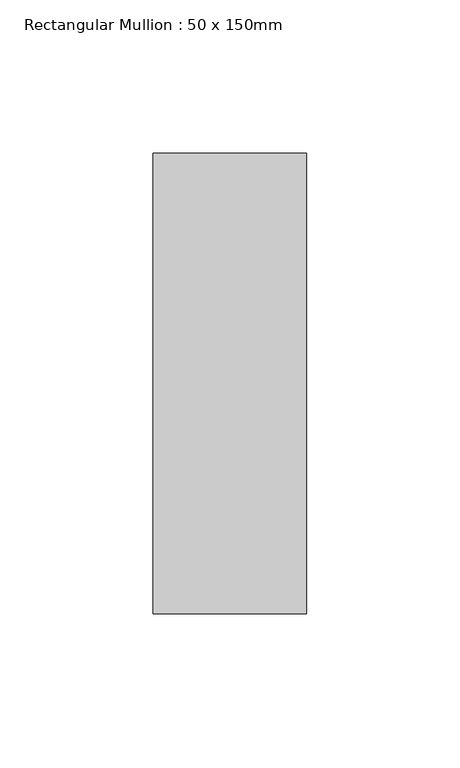
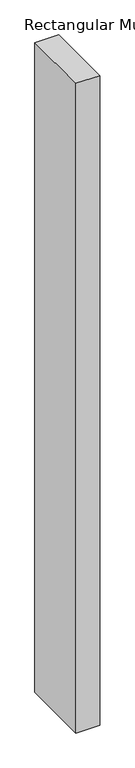
"""IFC4 building model written with IfcOpenShell, lengths in millimetres: member geometry, Rectangular Mullion : 50 x 150mm."""

import ifcopenshell
import ifcopenshell.guid

model = None  # the IFC model being written
_history = None  # IfcOwnerHistory: only IFC2X3 demands one
_inside = {}  # id of a spatial element -> (the spatial element, [elements in it])
_under = {}  # id of a project, library or spatial element -> (it, [spatial elements below it])
_declared = {}  # id of a project -> (the project, [libraries it declares])
_typed = {}  # id of a type object -> (the type object, [elements of that type])
_made_of = {}  # id of a material, layer set ... -> (it, [elements and type objects made of it])


def new_model(schema):
    """Start an empty IFC model of exactly this schema.

    Asked for "IFC4X3", IfcOpenShell would pick the latest addendum, in which some entities
    have other attributes; the version numbers below select the first issue.
    IFC2X3 requires an IfcOwnerHistory on every rooted entity: one is made here for all.
    """
    global model, _history
    if schema == "IFC4X3":
        model = ifcopenshell.file(schema_version=(4, 3, 0, 0))
    else:
        model = ifcopenshell.file(schema=schema)
    _inside.clear()
    _under.clear()
    _declared.clear()
    _typed.clear()
    _made_of.clear()
    _history = None
    if model.schema == "IFC2X3":
        org = make("IfcOrganization", Name="unknown")
        user = make(
            "IfcPersonAndOrganization",
            ThePerson=make("IfcPerson", FamilyName="unknown"),
            TheOrganization=org,
        )
        app = make(
            "IfcApplication",
            ApplicationDeveloper=org,
            Version="unknown",
            ApplicationFullName="unknown",
            ApplicationIdentifier="unknown",
        )
        _history = make(
            "IfcOwnerHistory",
            OwningUser=user,
            OwningApplication=app,
            ChangeAction="ADDED",
            CreationDate=0,
        )
    return model


def make(cls, **values):
    """One entity of the class cls with the attributes given. An attribute that is None is left unset."""
    return model.create_entity(
        cls, **{name: value for name, value in values.items() if value is not None}
    )


def rooted(cls, **values):
    """An entity with a GlobalId (a new one), such as an element, a storey or a relation."""
    return make(cls, GlobalId=ifcopenshell.guid.new(), OwnerHistory=_history, **values)


def si_unit(unit_type, name, prefix=None):
    """IfcSIUnit, for example si_unit("LENGTHUNIT", "METRE", prefix="MILLI")."""
    return make("IfcSIUnit", UnitType=unit_type, Prefix=prefix, Name=name)


def assignment(units):
    """IfcUnitAssignment: the units of a project."""
    return None if units is None else make("IfcUnitAssignment", Units=units)


def point(xyz):
    """IfcCartesianPoint."""
    return None if xyz is None else make("IfcCartesianPoint", Coordinates=xyz)


def direction(xyz):
    """IfcDirection."""
    return None if xyz is None else make("IfcDirection", DirectionRatios=xyz)


def frame(location, z_axis=None, x_axis=None):
    """IfcAxis2Placement3D, a coordinate frame: its origin and axes. An axis left out is left unset."""
    return make(
        "IfcAxis2Placement3D",
        Location=point(location),
        Axis=direction(z_axis),
        RefDirection=direction(x_axis),
    )


def origin():
    """The frame at (0, 0, 0) with its axes left unset."""
    return frame((0.0, 0.0, 0.0))


def place(relative_to, where):
    """IfcLocalPlacement: puts the frame where relative to a parent placement (None: the world)."""
    return make(
        "IfcLocalPlacement", PlacementRelTo=relative_to, RelativePlacement=where
    )


def context(
    kind, dimensions, precision=None, world=None, true_north=None, identifier=None
):
    """IfcGeometricRepresentationContext, for example the 3D "Model" context."""
    return make(
        "IfcGeometricRepresentationContext",
        ContextIdentifier=identifier,
        ContextType=kind,
        CoordinateSpaceDimension=dimensions,
        Precision=precision,
        WorldCoordinateSystem=world,
        TrueNorth=true_north,
    )


def project(units=None, contexts=None):
    """IfcProject with its units and contexts."""
    return rooted(
        "IfcProject",
        Name="project",
        RepresentationContexts=contexts,
        UnitsInContext=assignment(units),
    )


def spatial(cls, under=None, at=None, **own):
    """A site, building, storey or space (cls), placed at a placement, below another one or the project."""
    s = rooted(cls, ObjectPlacement=at, **own)
    if under is not None:
        _under.setdefault(under.id(), (under, []))[1].append(s)
    return s


def polyline(points):
    """IfcPolyline through the points."""
    return make("IfcPolyline", Points=[point(p) for p in points])


def outline(outer, holes=None, kind="AREA"):
    """IfcArbitraryClosedProfileDef: a profile drawn as a closed curve; with holes, ...WithVoids."""
    if holes is None:
        return make("IfcArbitraryClosedProfileDef", ProfileType=kind, OuterCurve=outer)
    return make(
        "IfcArbitraryProfileDefWithVoids",
        ProfileType=kind,
        OuterCurve=outer,
        InnerCurves=holes,
    )


def extrude(swept, where, along, depth):
    """IfcExtrudedAreaSolid: the profile swept, set in the frame where, extruded along a direction by depth."""
    return make(
        "IfcExtrudedAreaSolid",
        SweptArea=swept,
        Position=where,
        ExtrudedDirection=direction(along),
        Depth=depth,
    )


def shape(context_of_items, identifier, shape_type, items):
    """IfcShapeRepresentation: the items that make up one representation, for example the "Body"."""
    return make(
        "IfcShapeRepresentation",
        ContextOfItems=context_of_items,
        RepresentationIdentifier=identifier,
        RepresentationType=shape_type,
        Items=items,
    )


def source(mapping_origin, context_of_items, identifier, shape_type, items):
    """IfcRepresentationMap: a shape defined once, which mapped items show again and again."""
    return make(
        "IfcRepresentationMap",
        MappingOrigin=mapping_origin,
        MappedRepresentation=shape(context_of_items, identifier, shape_type, items),
    )


def transform(
    local_origin,
    x_axis=None,
    y_axis=None,
    z_axis=None,
    scale=None,
    scale2=None,
    scale3=None,
    uniform=True,
):
    """IfcCartesianTransformationOperator3D, or its non-uniform kind. x_axis, y_axis, z_axis: its Axis1, 2, 3."""
    if uniform:
        return make(
            "IfcCartesianTransformationOperator3D",
            Axis1=direction(x_axis),
            Axis2=direction(y_axis),
            LocalOrigin=point(local_origin),
            Scale=scale,
            Axis3=direction(z_axis),
        )
    return make(
        "IfcCartesianTransformationOperator3DnonUniform",
        Axis1=direction(x_axis),
        Axis2=direction(y_axis),
        LocalOrigin=point(local_origin),
        Scale=scale,
        Axis3=direction(z_axis),
        Scale2=scale2,
        Scale3=scale3,
    )


def mapped(mapping_source, mapping_target):
    """IfcMappedItem: shows the shape of a source again, moved by a transform."""
    return make(
        "IfcMappedItem", MappingSource=mapping_source, MappingTarget=mapping_target
    )


def made_of(thing, what):
    """Note that an element or type object is made of a material, layer set ...; save() writes the relation."""
    if what is not None:
        _made_of.setdefault(what.id(), (what, []))[1].append(thing)
    return thing


def element(
    cls,
    number,
    at=None,
    inside=None,
    cuts=None,
    type_object=None,
    material=None,
    context=None,
    identifier="Body",
    shape_type=None,
    held_by="IfcProductDefinitionShape",
    body=None,
    shapes=None,
    **own,
):
    """One element of the class cls, such as IfcWall. Its Tag is "e" and its number.

    at: its placement. inside: the storey or other place that contains it. cuts: it is an
    opening in that element (IfcRelVoidsElement). A single representation is given by context,
    identifier, shape_type and body (its items); several are given by shapes. held_by: the class
    of the entity that holds the representations. save() writes the other relations.
    """
    e = rooted(cls, Tag="e%d" % number, ObjectPlacement=at, **own)
    if body is not None:
        shapes = [shape(context, identifier, shape_type, body)]
    if shapes is not None:
        e.Representation = make(held_by, Representations=shapes)
    if inside is not None:
        _inside.setdefault(inside.id(), (inside, []))[1].append(e)
    if cuts is not None:
        rooted(
            "IfcRelVoidsElement", RelatingBuildingElement=cuts, RelatedOpeningElement=e
        )
    if type_object is not None:
        _typed.setdefault(type_object.id(), (type_object, []))[1].append(e)
    return made_of(e, material)


def aggregate(whole, parts):
    """IfcRelAggregates: a whole, such as a stair, and the parts it consists of."""
    return rooted("IfcRelAggregates", RelatingObject=whole, RelatedObjects=parts)


def save(model, path):
    """Write the relations noted so far, then the file.

    IfcRelAggregates (storeys below a building ...), IfcRelContainedInSpatialStructure (elements
    in a storey), IfcRelDefinesByType, IfcRelAssociatesMaterial and IfcRelDeclares: one each for
    every whole, place, type object, material and project.
    """
    for whole, parts in _under.values():
        aggregate(whole, parts)
    for where, things in _inside.values():
        rooted(
            "IfcRelContainedInSpatialStructure",
            RelatedElements=things,
            RelatingStructure=where,
        )
    for kind, things in _typed.values():
        rooted("IfcRelDefinesByType", RelatedObjects=things, RelatingType=kind)
    for what, things in _made_of.values():
        rooted("IfcRelAssociatesMaterial", RelatedObjects=things, RelatingMaterial=what)
    for by, libraries in _declared.values():
        rooted("IfcRelDeclares", RelatingContext=by, RelatedDefinitions=libraries)
    model.write(path)


def rectangular_mullion_50_x_150mm_a4200a9d(model_context):
    return source(origin(), model_context, "Body", "SweptSolid", [
        extrude(outline(polyline([(25.0, 75.0), (25.0, -75.0), (-25.0, -75.0), (-25.0, 75.0), (25.0, 75.0)])), frame((0.0, 0.0, -1450.1029933), z_axis=(0.0, 0.0, 1.0), x_axis=(1.0, 0.0, 0.0)), (0.0, 0.0, 1.0), 1450.1029933),
    ])


if __name__ == "__main__":
    model = new_model("IFC4")
    model_context = context("Model", 3, world=origin())
    ifc_project = project(units=[si_unit("LENGTHUNIT", "METRE", prefix="MILLI")], contexts=[model_context])
    site = spatial("IfcSite", under=ifc_project)
    building = spatial("IfcBuilding", under=site)
    placement = place(None, origin())
    rectangular_mullion_50_x_150mm_shape = rectangular_mullion_50_x_150mm_a4200a9d(model_context)
    element("IfcMember", 1, ObjectType="Rectangular Mullion : 50 x 150mm", at=placement, inside=building, context=model_context, shape_type="MappedRepresentation", body=[
        mapped(rectangular_mullion_50_x_150mm_shape, transform((0.0, 0.0, 0.0), x_axis=(1.0, 0.0, 0.0), y_axis=(0.0, 1.0, 0.0), z_axis=(0.0, 0.0, 1.0))),
    ])
    save(model, "model.ifc")

# Revit data of these elements
# Type "Rectangular Mullion : 50 x 150mm"
#   Keynote = "H11"
#   built-in parameter 1007304 = 0.492126 (stored number, unit not read)
#   built-in parameter 1007301 = 0.082021 (stored number, unit not read)
#   built-in parameter 1007300 = 0.082021 (stored number, unit not read)
# Element 1 (IfcMember, "Rectangular Mullion : 50 x 150mm")
#   Materials on its faces: "Aluminium"
# Materials
#   "Aluminium": class "Metal", colour RGB 247 247 247, transparency 0, Description = "Aluminium 6061", Cost = 0
